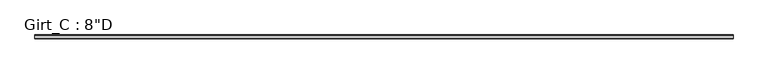
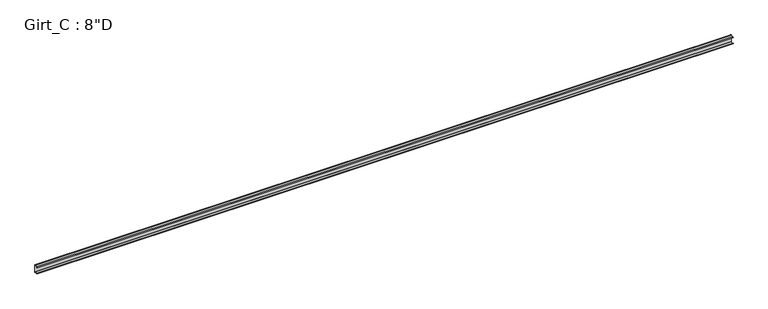
"""IFC4 building model written with IfcOpenShell, lengths in millimetres: beam geometry."""

import ifcopenshell
import ifcopenshell.guid

model = None  # the IFC model being written
_history = None  # IfcOwnerHistory: only IFC2X3 demands one
_inside = {}  # id of a spatial element -> (the spatial element, [elements in it])
_under = {}  # id of a project, library or spatial element -> (it, [spatial elements below it])
_declared = {}  # id of a project -> (the project, [libraries it declares])
_typed = {}  # id of a type object -> (the type object, [elements of that type])
_made_of = {}  # id of a material, layer set ... -> (it, [elements and type objects made of it])


def new_model(schema):
    """Start an empty IFC model of exactly this schema.

    Asked for "IFC4X3", IfcOpenShell would pick the latest addendum, in which some entities
    have other attributes; the version numbers below select the first issue.
    IFC2X3 requires an IfcOwnerHistory on every rooted entity: one is made here for all.
    """
    global model, _history
    if schema == "IFC4X3":
        model = ifcopenshell.file(schema_version=(4, 3, 0, 0))
    else:
        model = ifcopenshell.file(schema=schema)
    _inside.clear()
    _under.clear()
    _declared.clear()
    _typed.clear()
    _made_of.clear()
    _history = None
    if model.schema == "IFC2X3":
        org = make("IfcOrganization", Name="unknown")
        user = make(
            "IfcPersonAndOrganization",
            ThePerson=make("IfcPerson", FamilyName="unknown"),
            TheOrganization=org,
        )
        app = make(
            "IfcApplication",
            ApplicationDeveloper=org,
            Version="unknown",
            ApplicationFullName="unknown",
            ApplicationIdentifier="unknown",
        )
        _history = make(
            "IfcOwnerHistory",
            OwningUser=user,
            OwningApplication=app,
            ChangeAction="ADDED",
            CreationDate=0,
        )
    return model


def make(cls, **values):
    """One entity of the class cls with the attributes given. An attribute that is None is left unset."""
    return model.create_entity(
        cls, **{name: value for name, value in values.items() if value is not None}
    )


def rooted(cls, **values):
    """An entity with a GlobalId (a new one), such as an element, a storey or a relation."""
    return make(cls, GlobalId=ifcopenshell.guid.new(), OwnerHistory=_history, **values)


def si_unit(unit_type, name, prefix=None):
    """IfcSIUnit, for example si_unit("LENGTHUNIT", "METRE", prefix="MILLI")."""
    return make("IfcSIUnit", UnitType=unit_type, Prefix=prefix, Name=name)


def assignment(units):
    """IfcUnitAssignment: the units of a project."""
    return None if units is None else make("IfcUnitAssignment", Units=units)


def point(xyz):
    """IfcCartesianPoint."""
    return None if xyz is None else make("IfcCartesianPoint", Coordinates=xyz)


def direction(xyz):
    """IfcDirection."""
    return None if xyz is None else make("IfcDirection", DirectionRatios=xyz)


def frame(location, z_axis=None, x_axis=None):
    """IfcAxis2Placement3D, a coordinate frame: its origin and axes. An axis left out is left unset."""
    return make(
        "IfcAxis2Placement3D",
        Location=point(location),
        Axis=direction(z_axis),
        RefDirection=direction(x_axis),
    )


def frame_2d(location, x_axis=None):
    """IfcAxis2Placement2D, a coordinate frame in the plane: its origin and x axis."""
    return make(
        "IfcAxis2Placement2D", Location=point(location), RefDirection=direction(x_axis)
    )


def origin():
    """The frame at (0, 0, 0) with its axes left unset."""
    return frame((0.0, 0.0, 0.0))


def place(relative_to, where):
    """IfcLocalPlacement: puts the frame where relative to a parent placement (None: the world)."""
    return make(
        "IfcLocalPlacement", PlacementRelTo=relative_to, RelativePlacement=where
    )


def context(
    kind, dimensions, precision=None, world=None, true_north=None, identifier=None
):
    """IfcGeometricRepresentationContext, for example the 3D "Model" context."""
    return make(
        "IfcGeometricRepresentationContext",
        ContextIdentifier=identifier,
        ContextType=kind,
        CoordinateSpaceDimension=dimensions,
        Precision=precision,
        WorldCoordinateSystem=world,
        TrueNorth=true_north,
    )


def project(units=None, contexts=None):
    """IfcProject with its units and contexts."""
    return rooted(
        "IfcProject",
        Name="project",
        RepresentationContexts=contexts,
        UnitsInContext=assignment(units),
    )


def spatial(cls, under=None, at=None, **own):
    """A site, building, storey or space (cls), placed at a placement, below another one or the project."""
    s = rooted(cls, ObjectPlacement=at, **own)
    if under is not None:
        _under.setdefault(under.id(), (under, []))[1].append(s)
    return s


def polyline(points):
    """IfcPolyline through the points."""
    return make("IfcPolyline", Points=[point(p) for p in points])


def circle_curve(where, radius):
    """IfcCircle in the frame where."""
    return make("IfcCircle", Position=where, Radius=radius)


def trimmed(basis, trim1, trim2, sense, master):
    """IfcTrimmedCurve: the piece of a basis curve between two trims."""
    return make(
        "IfcTrimmedCurve",
        BasisCurve=basis,
        Trim1=trim1,
        Trim2=trim2,
        SenseAgreement=sense,
        MasterRepresentation=master,
    )


def segment(curve, same_sense, transition):
    """IfcCompositeCurveSegment."""
    return make(
        "IfcCompositeCurveSegment",
        Transition=transition,
        SameSense=same_sense,
        ParentCurve=curve,
    )


def composite_curve(segments, self_intersect=None):
    """IfcCompositeCurve: segments joined end to end."""
    return make("IfcCompositeCurve", Segments=segments, SelfIntersect=self_intersect)


def outline(outer, holes=None, kind="AREA"):
    """IfcArbitraryClosedProfileDef: a profile drawn as a closed curve; with holes, ...WithVoids."""
    if holes is None:
        return make("IfcArbitraryClosedProfileDef", ProfileType=kind, OuterCurve=outer)
    return make(
        "IfcArbitraryProfileDefWithVoids",
        ProfileType=kind,
        OuterCurve=outer,
        InnerCurves=holes,
    )


def extrude(swept, where, along, depth):
    """IfcExtrudedAreaSolid: the profile swept, set in the frame where, extruded along a direction by depth."""
    return make(
        "IfcExtrudedAreaSolid",
        SweptArea=swept,
        Position=where,
        ExtrudedDirection=direction(along),
        Depth=depth,
    )


def shape(context_of_items, identifier, shape_type, items):
    """IfcShapeRepresentation: the items that make up one representation, for example the "Body"."""
    return make(
        "IfcShapeRepresentation",
        ContextOfItems=context_of_items,
        RepresentationIdentifier=identifier,
        RepresentationType=shape_type,
        Items=items,
    )


def source(mapping_origin, context_of_items, identifier, shape_type, items):
    """IfcRepresentationMap: a shape defined once, which mapped items show again and again."""
    return make(
        "IfcRepresentationMap",
        MappingOrigin=mapping_origin,
        MappedRepresentation=shape(context_of_items, identifier, shape_type, items),
    )


def transform(
    local_origin,
    x_axis=None,
    y_axis=None,
    z_axis=None,
    scale=None,
    scale2=None,
    scale3=None,
    uniform=True,
):
    """IfcCartesianTransformationOperator3D, or its non-uniform kind. x_axis, y_axis, z_axis: its Axis1, 2, 3."""
    if uniform:
        return make(
            "IfcCartesianTransformationOperator3D",
            Axis1=direction(x_axis),
            Axis2=direction(y_axis),
            LocalOrigin=point(local_origin),
            Scale=scale,
            Axis3=direction(z_axis),
        )
    return make(
        "IfcCartesianTransformationOperator3DnonUniform",
        Axis1=direction(x_axis),
        Axis2=direction(y_axis),
        LocalOrigin=point(local_origin),
        Scale=scale,
        Axis3=direction(z_axis),
        Scale2=scale2,
        Scale3=scale3,
    )


def mapped(mapping_source, mapping_target):
    """IfcMappedItem: shows the shape of a source again, moved by a transform."""
    return make(
        "IfcMappedItem", MappingSource=mapping_source, MappingTarget=mapping_target
    )


def made_of(thing, what):
    """Note that an element or type object is made of a material, layer set ...; save() writes the relation."""
    if what is not None:
        _made_of.setdefault(what.id(), (what, []))[1].append(thing)
    return thing


def element(
    cls,
    number,
    at=None,
    inside=None,
    cuts=None,
    type_object=None,
    material=None,
    context=None,
    identifier="Body",
    shape_type=None,
    held_by="IfcProductDefinitionShape",
    body=None,
    shapes=None,
    **own,
):
    """One element of the class cls, such as IfcWall. Its Tag is "e" and its number.

    at: its placement. inside: the storey or other place that contains it. cuts: it is an
    opening in that element (IfcRelVoidsElement). A single representation is given by context,
    identifier, shape_type and body (its items); several are given by shapes. held_by: the class
    of the entity that holds the representations. save() writes the other relations.
    """
    e = rooted(cls, Tag="e%d" % number, ObjectPlacement=at, **own)
    if body is not None:
        shapes = [shape(context, identifier, shape_type, body)]
    if shapes is not None:
        e.Representation = make(held_by, Representations=shapes)
    if inside is not None:
        _inside.setdefault(inside.id(), (inside, []))[1].append(e)
    if cuts is not None:
        rooted(
            "IfcRelVoidsElement", RelatingBuildingElement=cuts, RelatedOpeningElement=e
        )
    if type_object is not None:
        _typed.setdefault(type_object.id(), (type_object, []))[1].append(e)
    return made_of(e, material)


def aggregate(whole, parts):
    """IfcRelAggregates: a whole, such as a stair, and the parts it consists of."""
    return rooted("IfcRelAggregates", RelatingObject=whole, RelatedObjects=parts)


def save(model, path):
    """Write the relations noted so far, then the file.

    IfcRelAggregates (storeys below a building ...), IfcRelContainedInSpatialStructure (elements
    in a storey), IfcRelDefinesByType, IfcRelAssociatesMaterial and IfcRelDeclares: one each for
    every whole, place, type object, material and project.
    """
    for whole, parts in _under.values():
        aggregate(whole, parts)
    for where, things in _inside.values():
        rooted(
            "IfcRelContainedInSpatialStructure",
            RelatedElements=things,
            RelatingStructure=where,
        )
    for kind, things in _typed.values():
        rooted("IfcRelDefinesByType", RelatedObjects=things, RelatingType=kind)
    for what, things in _made_of.values():
        rooted("IfcRelAssociatesMaterial", RelatedObjects=things, RelatingMaterial=what)
    for by, libraries in _declared.values():
        rooted("IfcRelDeclares", RelatingContext=by, RelatedDefinitions=libraries)
    model.write(path)


def beam_23314342(model_context):
    return source(origin(), model_context, "Body", "SweptSolid", [
        extrude(outline(composite_curve([segment(polyline([(-87.5109375, 101.6), (-3.3734375, 101.6)]), True, "CONTINUOUS"), segment(trimmed(circle_curve(frame_2d((-3.3734375, 96.8375)), 4.7625), [point((-3.3734375, 101.6))], [point((1.3890625, 96.8375))], False, "CARTESIAN"), True, "CONTINUOUS"), segment(polyline([(1.3890625, 96.8375), (1.3890625, -96.8375)]), True, "CONTINUOUS"), segment(trimmed(circle_curve(frame_2d((-3.3734375, -96.8375)), 4.7625), [point((1.3890625, -96.8375))], [point((-3.3734375, -101.6))], False, "CARTESIAN"), True, "CONTINUOUS"), segment(polyline([(-3.3734375, -101.6), (-87.5109375, -101.6), (-99.7792647, -86.979177), (-97.6510975, -85.1934327), (-86.2154765, -98.821875), (-3.2694106, -98.821875)]), True, "CONTINUOUS"), segment(trimmed(circle_curve(frame_2d((-3.3748024, -96.8389339)), 1.9857399), [point((-3.2694106, -98.821875))], [point((-1.3890625, -96.8389339))], True, "CARTESIAN"), True, "CONTINUOUS"), segment(polyline([(-1.3890625, -96.8389339), (-1.3890625, 96.8381931)]), True, "CONTINUOUS"), segment(trimmed(circle_curve(frame_2d((-3.3741066, 96.8381931)), 1.9850441), [point((-1.3890625, 96.8381931))], [point((-3.3005807, 98.821875))], True, "CARTESIAN"), True, "CONTINUOUS"), segment(polyline([(-3.3005807, 98.821875), (-86.2154765, 98.821875), (-97.6278742, 85.221109), (-99.7560415, 87.0068534), (-87.5109375, 101.6)]), True, "CONTINUOUS")], self_intersect=False)), frame((-9505.9373, 0.0, 0.0), z_axis=(1.0, 0.0, 0.0), x_axis=(0.0, 1.0, 0.0)), (0.0, 0.0, 1.0), 19069.939),
    ])


if __name__ == "__main__":
    model = new_model("IFC4")
    model_context = context("Model", 3, world=origin())
    ifc_project = project(units=[si_unit("LENGTHUNIT", "METRE", prefix="MILLI")], contexts=[model_context])
    site = spatial("IfcSite", under=ifc_project)
    building = spatial("IfcBuilding", under=site)
    placement = place(None, origin())
    beam_shape = beam_23314342(model_context)
    element("IfcBeam", 1, ObjectType="Girt_C : 8\"D", at=placement, inside=building, context=model_context, shape_type="MappedRepresentation", body=[
        mapped(beam_shape, transform((0.0, 0.0, 0.0), x_axis=(1.0, 0.0, 0.0), y_axis=(0.0, 1.0, 0.0), z_axis=(0.0, 0.0, 1.0))),
    ])
    save(model, "model.ifc")

# Revit data of these elements
# Type "Girt_C : 8\"D"
#   half leg = 0' - 1 3/4"
#   Web_Thickness = 0' - 0 7/64"
#   Length [instance default] = 10' - 0"
#   Leg_1 = 0' - 3 1/2"
#   Height = 0' - 8"
#   Structural Material [instance default] = none
# Element 1 (IfcBeam, "Girt_C : 8\"D")
#   Materials on its faces: "CEE' SECTION (8.0x3.5C - SEE STRUCT. DWGS)"
# Materials
#   "CEE' SECTION (8.0x3.5C - SEE STRUCT. DWGS)": class "Metal", colour RGB 137 146 153, transparency 0, Description = "Steel, mill finish", Cost = 0
